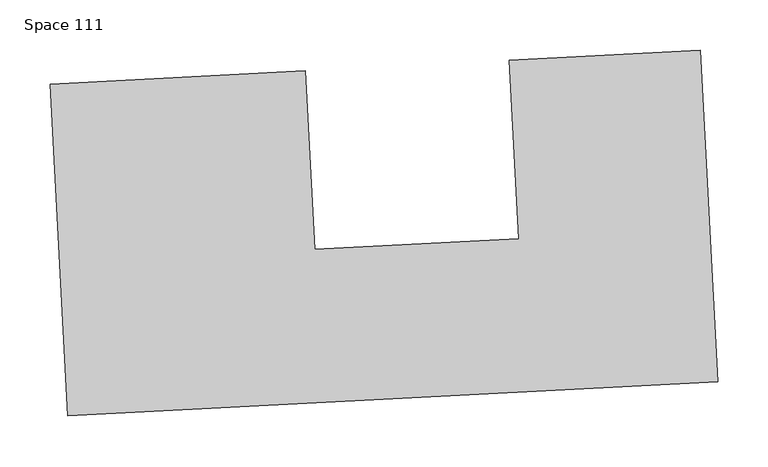
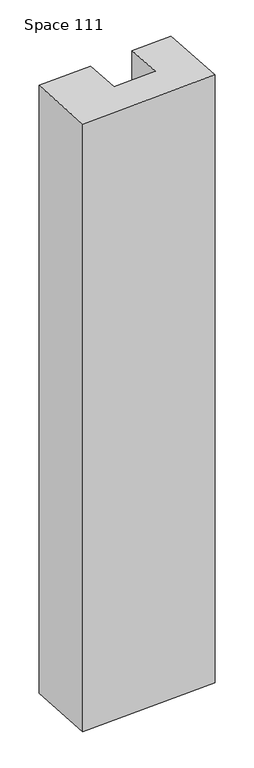
"""IFC4 building model written with IfcOpenShell, lengths in millimetres: proxy geometry, Space 111."""

from ifc_helpers import new_model, si_unit, origin, origin_with_axes, place, context, project, spatial, polyline, outline, extrude, source, transform, mapped, element, save


def space_111_51e88c58(model_context):
    return source(origin(), model_context, "Body", "SweptSolid", [
        extrude(outline(polyline([(6390.340635, -35021.8968987), (6373.0593022, -34692.1494264), (6626.7112041, -34678.8560935), (6636.0165371, -34856.4124248), (6838.9380585, -34845.7777585), (6829.6327255, -34668.2214272), (7019.8716519, -34658.2514275), (7037.1529846, -34987.9988999), (6390.340635, -35021.8968987)])), origin_with_axes(), (0.0, 0.0, 1.0), 3048.0),
    ])


if __name__ == "__main__":
    model = new_model("IFC4")
    model_context = context("Model", 3, world=origin())
    ifc_project = project(units=[si_unit("LENGTHUNIT", "METRE", prefix="MILLI")], contexts=[model_context])
    site = spatial("IfcSite", under=ifc_project)
    building = spatial("IfcBuilding", under=site)
    placement = place(None, origin())
    space_111_shape = space_111_51e88c58(model_context)
    element("IfcBuildingElementProxy", 1, Name="Space 111", ObjectType="Space 111", at=placement, inside=building, context=model_context, shape_type="MappedRepresentation", body=[
        mapped(space_111_shape, transform((0.0, 0.0, 0.0), x_axis=(1.0, 0.0, 0.0), y_axis=(0.0, 1.0, 0.0), z_axis=(0.0, 0.0, 1.0))),
    ])
    save(model, "model.ifc")

# Revit data of these elements
# Element 1 (IfcBuildingElementProxy, "Space 111")
#   Materials on its faces: "Render Material 255-255-255"
# Materials
#   "Render Material 255-255-255": class "Unassigned", colour RGB 255 255 255, transparency 0
